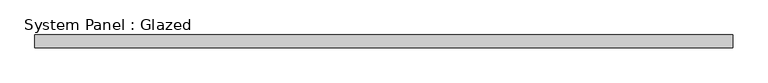
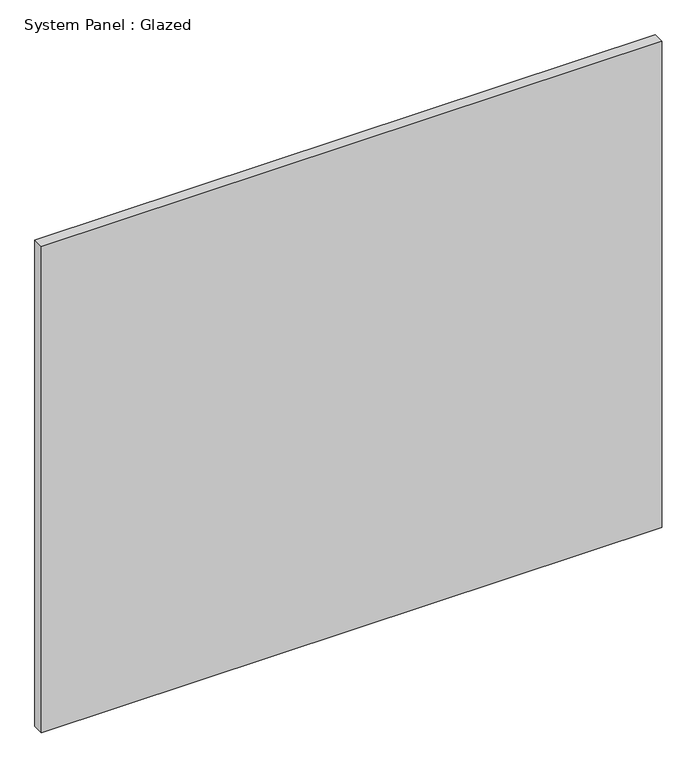
"""IFC4 building model written with IfcOpenShell, lengths in millimetres: plate geometry, System Panel : Glazed."""

import ifcopenshell
import ifcopenshell.guid

model = None  # the IFC model being written
_history = None  # IfcOwnerHistory: only IFC2X3 demands one
_inside = {}  # id of a spatial element -> (the spatial element, [elements in it])
_under = {}  # id of a project, library or spatial element -> (it, [spatial elements below it])
_declared = {}  # id of a project -> (the project, [libraries it declares])
_typed = {}  # id of a type object -> (the type object, [elements of that type])
_made_of = {}  # id of a material, layer set ... -> (it, [elements and type objects made of it])


def new_model(schema):
    """Start an empty IFC model of exactly this schema.

    Asked for "IFC4X3", IfcOpenShell would pick the latest addendum, in which some entities
    have other attributes; the version numbers below select the first issue.
    IFC2X3 requires an IfcOwnerHistory on every rooted entity: one is made here for all.
    """
    global model, _history
    if schema == "IFC4X3":
        model = ifcopenshell.file(schema_version=(4, 3, 0, 0))
    else:
        model = ifcopenshell.file(schema=schema)
    _inside.clear()
    _under.clear()
    _declared.clear()
    _typed.clear()
    _made_of.clear()
    _history = None
    if model.schema == "IFC2X3":
        org = make("IfcOrganization", Name="unknown")
        user = make(
            "IfcPersonAndOrganization",
            ThePerson=make("IfcPerson", FamilyName="unknown"),
            TheOrganization=org,
        )
        app = make(
            "IfcApplication",
            ApplicationDeveloper=org,
            Version="unknown",
            ApplicationFullName="unknown",
            ApplicationIdentifier="unknown",
        )
        _history = make(
            "IfcOwnerHistory",
            OwningUser=user,
            OwningApplication=app,
            ChangeAction="ADDED",
            CreationDate=0,
        )
    return model


def make(cls, **values):
    """One entity of the class cls with the attributes given. An attribute that is None is left unset."""
    return model.create_entity(
        cls, **{name: value for name, value in values.items() if value is not None}
    )


def rooted(cls, **values):
    """An entity with a GlobalId (a new one), such as an element, a storey or a relation."""
    return make(cls, GlobalId=ifcopenshell.guid.new(), OwnerHistory=_history, **values)


def si_unit(unit_type, name, prefix=None):
    """IfcSIUnit, for example si_unit("LENGTHUNIT", "METRE", prefix="MILLI")."""
    return make("IfcSIUnit", UnitType=unit_type, Prefix=prefix, Name=name)


def assignment(units):
    """IfcUnitAssignment: the units of a project."""
    return None if units is None else make("IfcUnitAssignment", Units=units)


def point(xyz):
    """IfcCartesianPoint."""
    return None if xyz is None else make("IfcCartesianPoint", Coordinates=xyz)


def direction(xyz):
    """IfcDirection."""
    return None if xyz is None else make("IfcDirection", DirectionRatios=xyz)


def frame(location, z_axis=None, x_axis=None):
    """IfcAxis2Placement3D, a coordinate frame: its origin and axes. An axis left out is left unset."""
    return make(
        "IfcAxis2Placement3D",
        Location=point(location),
        Axis=direction(z_axis),
        RefDirection=direction(x_axis),
    )


def origin():
    """The frame at (0, 0, 0) with its axes left unset."""
    return frame((0.0, 0.0, 0.0))


def origin_with_axes():
    """The frame at (0, 0, 0) with the z axis (0, 0, 1) and the x axis (1, 0, 0) written out."""
    return frame((0.0, 0.0, 0.0), z_axis=(0.0, 0.0, 1.0), x_axis=(1.0, 0.0, 0.0))


def place(relative_to, where):
    """IfcLocalPlacement: puts the frame where relative to a parent placement (None: the world)."""
    return make(
        "IfcLocalPlacement", PlacementRelTo=relative_to, RelativePlacement=where
    )


def context(
    kind, dimensions, precision=None, world=None, true_north=None, identifier=None
):
    """IfcGeometricRepresentationContext, for example the 3D "Model" context."""
    return make(
        "IfcGeometricRepresentationContext",
        ContextIdentifier=identifier,
        ContextType=kind,
        CoordinateSpaceDimension=dimensions,
        Precision=precision,
        WorldCoordinateSystem=world,
        TrueNorth=true_north,
    )


def project(units=None, contexts=None):
    """IfcProject with its units and contexts."""
    return rooted(
        "IfcProject",
        Name="project",
        RepresentationContexts=contexts,
        UnitsInContext=assignment(units),
    )


def spatial(cls, under=None, at=None, **own):
    """A site, building, storey or space (cls), placed at a placement, below another one or the project."""
    s = rooted(cls, ObjectPlacement=at, **own)
    if under is not None:
        _under.setdefault(under.id(), (under, []))[1].append(s)
    return s


def polyline(points):
    """IfcPolyline through the points."""
    return make("IfcPolyline", Points=[point(p) for p in points])


def outline(outer, holes=None, kind="AREA"):
    """IfcArbitraryClosedProfileDef: a profile drawn as a closed curve; with holes, ...WithVoids."""
    if holes is None:
        return make("IfcArbitraryClosedProfileDef", ProfileType=kind, OuterCurve=outer)
    return make(
        "IfcArbitraryProfileDefWithVoids",
        ProfileType=kind,
        OuterCurve=outer,
        InnerCurves=holes,
    )


def extrude(swept, where, along, depth):
    """IfcExtrudedAreaSolid: the profile swept, set in the frame where, extruded along a direction by depth."""
    return make(
        "IfcExtrudedAreaSolid",
        SweptArea=swept,
        Position=where,
        ExtrudedDirection=direction(along),
        Depth=depth,
    )


def shape(context_of_items, identifier, shape_type, items):
    """IfcShapeRepresentation: the items that make up one representation, for example the "Body"."""
    return make(
        "IfcShapeRepresentation",
        ContextOfItems=context_of_items,
        RepresentationIdentifier=identifier,
        RepresentationType=shape_type,
        Items=items,
    )


def source(mapping_origin, context_of_items, identifier, shape_type, items):
    """IfcRepresentationMap: a shape defined once, which mapped items show again and again."""
    return make(
        "IfcRepresentationMap",
        MappingOrigin=mapping_origin,
        MappedRepresentation=shape(context_of_items, identifier, shape_type, items),
    )


def transform(
    local_origin,
    x_axis=None,
    y_axis=None,
    z_axis=None,
    scale=None,
    scale2=None,
    scale3=None,
    uniform=True,
):
    """IfcCartesianTransformationOperator3D, or its non-uniform kind. x_axis, y_axis, z_axis: its Axis1, 2, 3."""
    if uniform:
        return make(
            "IfcCartesianTransformationOperator3D",
            Axis1=direction(x_axis),
            Axis2=direction(y_axis),
            LocalOrigin=point(local_origin),
            Scale=scale,
            Axis3=direction(z_axis),
        )
    return make(
        "IfcCartesianTransformationOperator3DnonUniform",
        Axis1=direction(x_axis),
        Axis2=direction(y_axis),
        LocalOrigin=point(local_origin),
        Scale=scale,
        Axis3=direction(z_axis),
        Scale2=scale2,
        Scale3=scale3,
    )


def mapped(mapping_source, mapping_target):
    """IfcMappedItem: shows the shape of a source again, moved by a transform."""
    return make(
        "IfcMappedItem", MappingSource=mapping_source, MappingTarget=mapping_target
    )


def made_of(thing, what):
    """Note that an element or type object is made of a material, layer set ...; save() writes the relation."""
    if what is not None:
        _made_of.setdefault(what.id(), (what, []))[1].append(thing)
    return thing


def element(
    cls,
    number,
    at=None,
    inside=None,
    cuts=None,
    type_object=None,
    material=None,
    context=None,
    identifier="Body",
    shape_type=None,
    held_by="IfcProductDefinitionShape",
    body=None,
    shapes=None,
    **own,
):
    """One element of the class cls, such as IfcWall. Its Tag is "e" and its number.

    at: its placement. inside: the storey or other place that contains it. cuts: it is an
    opening in that element (IfcRelVoidsElement). A single representation is given by context,
    identifier, shape_type and body (its items); several are given by shapes. held_by: the class
    of the entity that holds the representations. save() writes the other relations.
    """
    e = rooted(cls, Tag="e%d" % number, ObjectPlacement=at, **own)
    if body is not None:
        shapes = [shape(context, identifier, shape_type, body)]
    if shapes is not None:
        e.Representation = make(held_by, Representations=shapes)
    if inside is not None:
        _inside.setdefault(inside.id(), (inside, []))[1].append(e)
    if cuts is not None:
        rooted(
            "IfcRelVoidsElement", RelatingBuildingElement=cuts, RelatedOpeningElement=e
        )
    if type_object is not None:
        _typed.setdefault(type_object.id(), (type_object, []))[1].append(e)
    return made_of(e, material)


def aggregate(whole, parts):
    """IfcRelAggregates: a whole, such as a stair, and the parts it consists of."""
    return rooted("IfcRelAggregates", RelatingObject=whole, RelatedObjects=parts)


def save(model, path):
    """Write the relations noted so far, then the file.

    IfcRelAggregates (storeys below a building ...), IfcRelContainedInSpatialStructure (elements
    in a storey), IfcRelDefinesByType, IfcRelAssociatesMaterial and IfcRelDeclares: one each for
    every whole, place, type object, material and project.
    """
    for whole, parts in _under.values():
        aggregate(whole, parts)
    for where, things in _inside.values():
        rooted(
            "IfcRelContainedInSpatialStructure",
            RelatedElements=things,
            RelatingStructure=where,
        )
    for kind, things in _typed.values():
        rooted("IfcRelDefinesByType", RelatedObjects=things, RelatingType=kind)
    for what, things in _made_of.values():
        rooted("IfcRelAssociatesMaterial", RelatedObjects=things, RelatingMaterial=what)
    for by, libraries in _declared.values():
        rooted("IfcRelDeclares", RelatingContext=by, RelatedDefinitions=libraries)
    model.write(path)


def system_panel_glazed_d25bfe26(model_context):
    return source(origin(), model_context, "Body", "SweptSolid", [
        extrude(outline(polyline([(697.4416668, -44.45), (-697.4416668, -44.45), (-697.4416668, -19.05), (697.4416668, -19.05), (697.4416668, -44.45)])), origin_with_axes(), (0.0, 0.0, 1.0), 1155.7),
    ])


if __name__ == "__main__":
    model = new_model("IFC4")
    model_context = context("Model", 3, world=origin())
    ifc_project = project(units=[si_unit("LENGTHUNIT", "METRE", prefix="MILLI")], contexts=[model_context])
    site = spatial("IfcSite", under=ifc_project)
    building = spatial("IfcBuilding", under=site)
    placement = place(None, origin())
    system_panel_glazed_shape = system_panel_glazed_d25bfe26(model_context)
    element("IfcPlate", 1, ObjectType="System Panel : Glazed", at=placement, inside=building, context=model_context, shape_type="MappedRepresentation", body=[
        mapped(system_panel_glazed_shape, transform((0.0, 0.0, 0.0), x_axis=(1.0, 0.0, 0.0), y_axis=(0.0, 1.0, 0.0), z_axis=(0.0, 0.0, 1.0))),
    ])
    save(model, "model.ifc")

# Revit data of these elements
# Type "System Panel : Glazed"
#   Construction Type Id = "GSP4R"
#   Analytic Construction = "1/8 in Pilkington single glazing"
#   Visual Light Transmittance = 0.9
#   Solar Heat Gain Coefficient = 0.86
#   Heat Transfer Coefficient (U) = 1.18115 BTU/(h·ft²·°F)
#   Define Thermal Properties by = 1
# Element 1 (IfcPlate, "System Panel : Glazed")
#   Materials on its faces: "Glass"
# Materials
#   "Glass": class "Glass", colour RGB 0 128 192, transparency 0.75, Description = "Soda Lime Glass", Cost = 0
